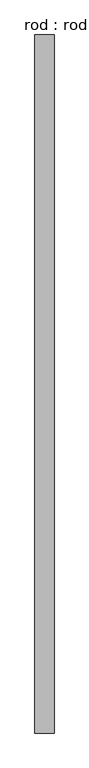
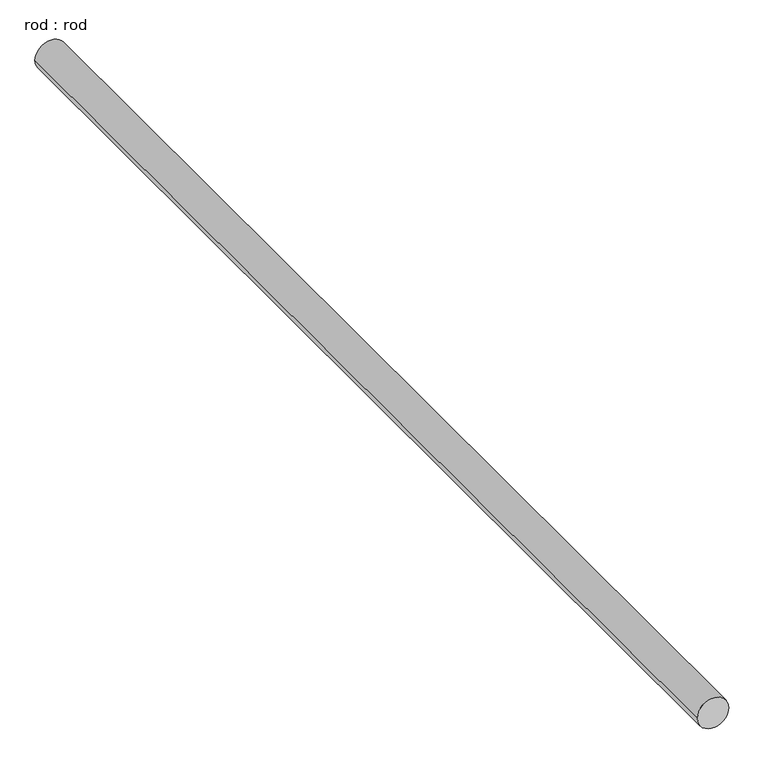
"""IFC4 building model written with IfcOpenShell, lengths in millimetres: proxy geometry, rod : rod."""

from ifc_helpers import new_model, si_unit, point, frame, frame_2d, origin, place, context, project, spatial, circle_curve, trimmed, segment, composite_curve, outline, extrude, source, transform, mapped, element, save


def rod_rod_e8ff26a9(model_context):
    return source(origin(), model_context, "Body", "SweptSolid", [
        extrude(outline(composite_curve([segment(trimmed(circle_curve(frame_2d((0.0108462, 0.0)), 200.0), [point((0.0108462, 200.0))], [point((0.0108462, -200.0))], False, "CARTESIAN"), True, "CONTINUOUS"), segment(trimmed(circle_curve(frame_2d((0.0108462, 0.0)), 200.0), [point((0.0108462, -200.0))], [point((0.0108462, 200.0))], False, "CARTESIAN"), True, "CONTINUOUS")], self_intersect=False)), frame((0.0, -3192.9856704, 0.0), z_axis=(0.0, 1.0, 0.0), x_axis=(0.0, 0.0, 1.0)), (0.0, 0.0, 1.0), 14571.4285714),
    ])


if __name__ == "__main__":
    model = new_model("IFC4")
    model_context = context("Model", 3, world=origin())
    ifc_project = project(units=[si_unit("LENGTHUNIT", "METRE", prefix="MILLI")], contexts=[model_context])
    site = spatial("IfcSite", under=ifc_project)
    building = spatial("IfcBuilding", under=site)
    placement = place(None, origin())
    rod_rod_shape = rod_rod_e8ff26a9(model_context)
    element("IfcBuildingElementProxy", 1, Name="rod : rod", ObjectType="rod : rod", at=placement, inside=building, context=model_context, shape_type="MappedRepresentation", body=[
        mapped(rod_rod_shape, transform((0.0, 0.0, 0.0), x_axis=(1.0, 0.0, 0.0), y_axis=(0.0, 1.0, 0.0), z_axis=(0.0, 0.0, 1.0))),
    ])
    save(model, "model.ifc")

# Revit data of these elements
# Type "rod : rod"
#   Default Elevation = 0
